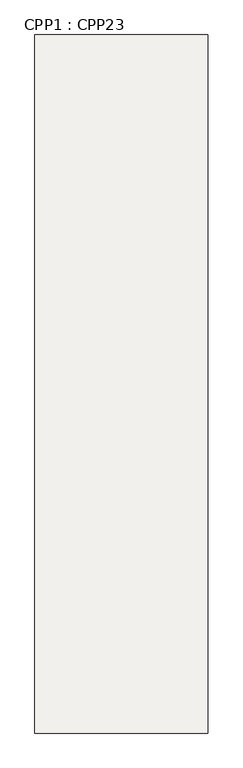
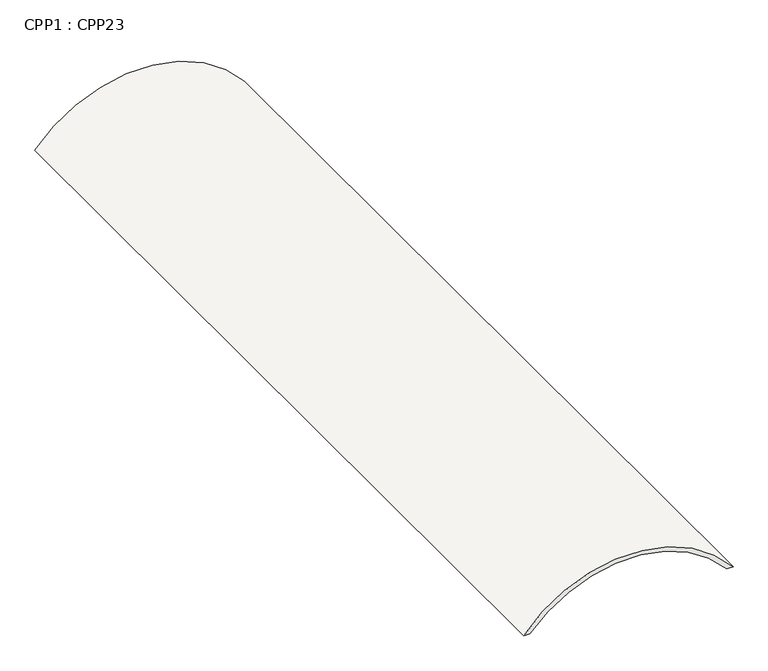
"""IFC4 building model written with IfcOpenShell, lengths in millimetres: slab geometry, CPP1 : CPP23."""

from ifc_helpers import new_model, si_unit, point, frame, frame_2d, origin, place, context, project, spatial, polyline, circle_curve, trimmed, segment, composite_curve, outline, extrude, source, transform, mapped, element, save


def cpp1_cpp23_fabdbfc1(model_context):
    return source(origin(), model_context, "Body", "SweptSolid", [
        extrude(outline(composite_curve([segment(polyline([(14620.0, 35333.2245514), (14620.0, 35483.2245514)]), True, "CONTINUOUS"), segment(trimmed(circle_curve(frame_2d((12603.2870371, 37833.2245514)), 3096.7129629), [point((14620.0, 35483.2245514))], [point((14620.0, 40183.2245513))], True, "CARTESIAN"), True, "CONTINUOUS"), segment(polyline([(14620.0, 40183.2245513), (14620.0, 40333.2245513)]), True, "CONTINUOUS"), segment(trimmed(circle_curve(frame_2d((12561.6949153, 37833.2245514)), 3238.3050847), [point((14620.0, 40333.2245513))], [point((14620.0, 35333.2245514))], False, "CARTESIAN"), True, "CONTINUOUS")], self_intersect=False)), frame((0.0, -100.2551788, 0.0), z_axis=(0.0, 1.0, 0.0), x_axis=(0.0, 0.0, 1.0)), (0.0, 0.0, 1.0), 20199.9999981),
    ])


if __name__ == "__main__":
    model = new_model("IFC4")
    model_context = context("Model", 3, world=origin())
    ifc_project = project(units=[si_unit("LENGTHUNIT", "METRE", prefix="MILLI")], contexts=[model_context])
    site = spatial("IfcSite", under=ifc_project)
    building = spatial("IfcBuilding", under=site)
    placement = place(None, origin())
    cpp1_cpp23_shape = cpp1_cpp23_fabdbfc1(model_context)
    element("IfcSlab", 1, ObjectType="CPP1 : CPP23", at=placement, inside=building, context=model_context, shape_type="MappedRepresentation", body=[
        mapped(cpp1_cpp23_shape, transform((0.0, 0.0, 0.0), x_axis=(1.0, 0.0, 0.0), y_axis=(0.0, 1.0, 0.0), z_axis=(0.0, 0.0, 1.0))),
    ])
    save(model, "model.ifc")

# Revit data of these elements
# Element 1 (IfcSlab, "CPP1 : CPP23")
#   Materials on its faces: "Concrete, RC"
# Materials
#   "Concrete, RC": class "Concrete", colour RGB 128 128 128, transparency 0, Description = "Cast-in-place concrete", Cost = 0
